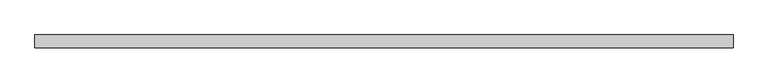
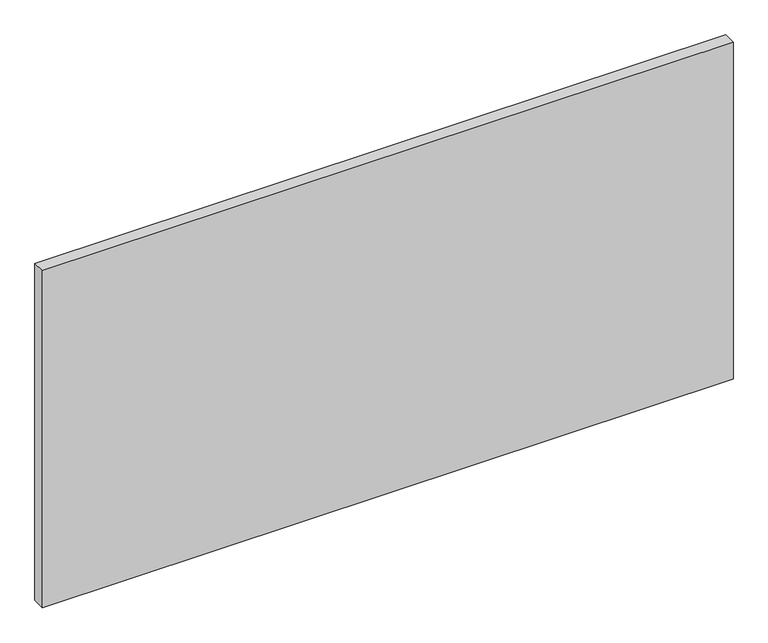
"""IFC4 building model written with IfcOpenShell, lengths in millimetres: plate geometry, システム パネル : ガラス."""

from ifc_helpers import new_model, si_unit, origin, origin_with_axes, place, context, project, spatial, polyline, outline, extrude, source, transform, mapped, element, save


def plate_0eebf7e9(model_context):
    return source(origin(), model_context, "Body", "SweptSolid", [
        extrude(outline(polyline([(678.1250001, 24.5), (-678.1250001, 24.5), (-678.1250001, 49.5), (678.1250001, 49.5), (678.1250001, 24.5)])), origin_with_axes(), (0.0, 0.0, 1.0), 700.0),
    ])


if __name__ == "__main__":
    model = new_model("IFC4")
    model_context = context("Model", 3, world=origin())
    ifc_project = project(units=[si_unit("LENGTHUNIT", "METRE", prefix="MILLI")], contexts=[model_context])
    site = spatial("IfcSite", under=ifc_project)
    building = spatial("IfcBuilding", under=site)
    placement = place(None, origin())
    plate_shape = plate_0eebf7e9(model_context)
    element("IfcPlate", 1, ObjectType="システム パネル : ガラス", at=placement, inside=building, context=model_context, shape_type="MappedRepresentation", body=[
        mapped(plate_shape, transform((0.0, 0.0, 0.0), x_axis=(1.0, 0.0, 0.0), y_axis=(0.0, 1.0, 0.0), z_axis=(0.0, 0.0, 1.0))),
    ])
    save(model, "model.ifc")

# Revit data of these elements
# Type "システム パネル : ガラス"
#   Construction Type Id = "GSP4R"
#   Analytic Construction = "1/8 インチ ピルキントン一重ガラス"
#   Visual Light Transmittance = 0.9
#   Solar Heat Gain Coefficient = 0.86
#   Heat Transfer Coefficient (U) = 6.7069 W/(m²·K)
# Element 1 (IfcPlate, "システム パネル : ガラス")
#   Materials on its faces: "ガラス - 透明"
# Materials
#   "ガラス - 透明": class "ガラス", colour RGB 0 128 192, transparency 0.9, Cost = 0
